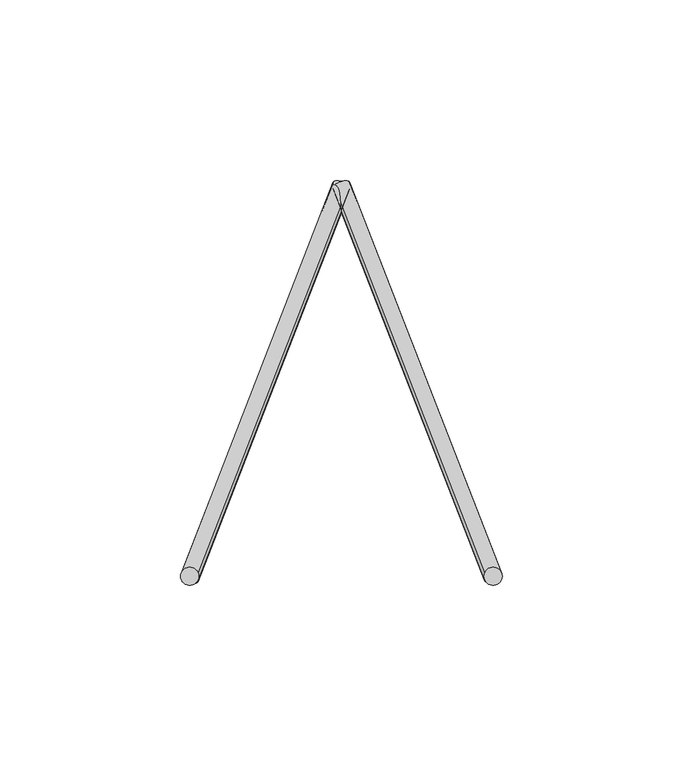
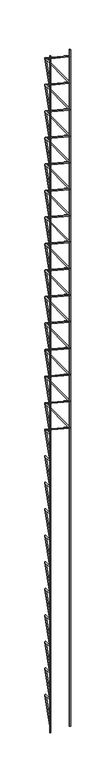
"""IFC4 building model written with IfcOpenShell, lengths in millimetres: proxy geometry, Pre-fab. (Vigota 1 - Pano 3)."""

from ifc_helpers import new_model, si_unit, point, frame, frame_2d, origin, origin_with_axes, origin_2d, place, context, project, spatial, circle_curve, trimmed, segment, composite_curve, outline, extrude, source, transform, mapped, element, save


def structural_framing_81210333(model_context):
    return source(origin(), model_context, "Body", "SweptSolid", [
        extrude(outline(composite_curve([segment(trimmed(circle_curve(origin_2d(), 2.5), [point((2.5, 0.0))], [point((-2.5, 0.0))], False, "CARTESIAN"), True, "CONTINUOUS"), segment(trimmed(circle_curve(origin_2d(), 2.5), [point((-2.5, 0.0))], [point((2.5, 0.0))], False, "CARTESIAN"), True, "CONTINUOUS")], self_intersect=False)), frame((-42.0, 108.0, 1289.500535), z_axis=(0.3218603428886276, -0.8276408817707567, 0.4598004898837537), x_axis=(0.8192319205108605, -3.936835275445103e-11, -0.5734623443750141)), (0.0, 0.0, 1.0), 130.491379),
        extrude(outline(composite_curve([segment(trimmed(circle_curve(origin_2d(), 2.5), [point((2.5, 0.0))], [point((-2.5, 0.0))], False, "CARTESIAN"), True, "CONTINUOUS"), segment(trimmed(circle_curve(origin_2d(), 2.5), [point((-2.5, 0.0))], [point((2.5, 0.0))], False, "CARTESIAN"), True, "CONTINUOUS")], self_intersect=False)), frame((0.0, 0.0, 1349.500535), z_axis=(-0.3218603428886276, 0.8276408817707567, 0.4598004898837537), x_axis=(0.8192319205108605, -3.936835275445103e-11, 0.5734623443750141)), (0.0, 0.0, 1.0), 130.491379),
        extrude(outline(composite_curve([segment(trimmed(circle_curve(origin_2d(), 2.5), [point((2.5, 0.0))], [point((-2.5, 0.0))], False, "CARTESIAN"), True, "CONTINUOUS"), segment(trimmed(circle_curve(origin_2d(), 2.5), [point((-2.5, 0.0))], [point((2.5, 0.0))], False, "CARTESIAN"), True, "CONTINUOUS")], self_intersect=False)), frame((-42.0, 108.0, 1409.500535), z_axis=(0.3218603428886276, -0.8276408817707567, 0.4598004898837537), x_axis=(0.8192319205108605, -3.936835275445103e-11, -0.5734623443750141)), (0.0, 0.0, 1.0), 130.491379),
        extrude(outline(composite_curve([segment(trimmed(circle_curve(origin_2d(), 2.5), [point((2.5, 0.0))], [point((-2.5, 0.0))], False, "CARTESIAN"), True, "CONTINUOUS"), segment(trimmed(circle_curve(origin_2d(), 2.5), [point((-2.5, 0.0))], [point((2.5, 0.0))], False, "CARTESIAN"), True, "CONTINUOUS")], self_intersect=False)), frame((0.0, 0.0, 1469.500535), z_axis=(-0.3218603428886276, 0.8276408817707567, 0.4598004898837537), x_axis=(0.8192319205108605, -3.936835275445103e-11, 0.5734623443750141)), (0.0, 0.0, 1.0), 130.491379),
        extrude(outline(composite_curve([segment(trimmed(circle_curve(origin_2d(), 2.5), [point((2.5, 0.0))], [point((-2.5, 0.0))], False, "CARTESIAN"), True, "CONTINUOUS"), segment(trimmed(circle_curve(origin_2d(), 2.5), [point((-2.5, 0.0))], [point((2.5, 0.0))], False, "CARTESIAN"), True, "CONTINUOUS")], self_intersect=False)), frame((-42.0, 108.0, 1529.500535), z_axis=(0.3218603428886276, -0.8276408817707567, 0.4598004898837537), x_axis=(0.8192319205108605, -3.936835275445103e-11, -0.5734623443750141)), (0.0, 0.0, 1.0), 130.491379),
        extrude(outline(composite_curve([segment(trimmed(circle_curve(origin_2d(), 2.5), [point((2.5, 0.0))], [point((-2.5, 0.0))], False, "CARTESIAN"), True, "CONTINUOUS"), segment(trimmed(circle_curve(origin_2d(), 2.5), [point((-2.5, 0.0))], [point((2.5, 0.0))], False, "CARTESIAN"), True, "CONTINUOUS")], self_intersect=False)), frame((0.0, 0.0, 1589.500535), z_axis=(-0.3218603428886276, 0.8276408817707567, 0.4598004898837537), x_axis=(0.8192319205108605, -3.936835275445103e-11, 0.5734623443750141)), (0.0, 0.0, 1.0), 130.491379),
        extrude(outline(composite_curve([segment(trimmed(circle_curve(origin_2d(), 2.5), [point((2.5, 0.0))], [point((-2.5, 0.0))], False, "CARTESIAN"), True, "CONTINUOUS"), segment(trimmed(circle_curve(origin_2d(), 2.5), [point((-2.5, 0.0))], [point((2.5, 0.0))], False, "CARTESIAN"), True, "CONTINUOUS")], self_intersect=False)), frame((-42.0, 108.0, 1649.500535), z_axis=(0.3218603428886276, -0.8276408817707567, 0.4598004898837537), x_axis=(0.8192319205108605, -3.936835275445103e-11, -0.5734623443750141)), (0.0, 0.0, 1.0), 130.491379),
        extrude(outline(composite_curve([segment(trimmed(circle_curve(origin_2d(), 2.5), [point((2.5, 0.0))], [point((-2.5, 0.0))], False, "CARTESIAN"), True, "CONTINUOUS"), segment(trimmed(circle_curve(origin_2d(), 2.5), [point((-2.5, 0.0))], [point((2.5, 0.0))], False, "CARTESIAN"), True, "CONTINUOUS")], self_intersect=False)), frame((0.0, 0.0, 1709.500535), z_axis=(-0.3218603428886276, 0.8276408817707567, 0.4598004898837537), x_axis=(0.8192319205108605, -3.936835275445103e-11, 0.5734623443750141)), (0.0, 0.0, 1.0), 130.491379),
        extrude(outline(composite_curve([segment(trimmed(circle_curve(origin_2d(), 2.5), [point((2.5, 0.0))], [point((-2.5, 0.0))], False, "CARTESIAN"), True, "CONTINUOUS"), segment(trimmed(circle_curve(origin_2d(), 2.5), [point((-2.5, 0.0))], [point((2.5, 0.0))], False, "CARTESIAN"), True, "CONTINUOUS")], self_intersect=False)), frame((-42.0, 108.0, 1769.500535), z_axis=(0.3218603428886276, -0.8276408817707567, 0.4598004898837537), x_axis=(0.8192319205108605, -3.936835275445103e-11, -0.5734623443750141)), (0.0, 0.0, 1.0), 130.491379),
        extrude(outline(composite_curve([segment(trimmed(circle_curve(origin_2d(), 2.5), [point((2.5, 0.0))], [point((-2.5, 0.0))], False, "CARTESIAN"), True, "CONTINUOUS"), segment(trimmed(circle_curve(origin_2d(), 2.5), [point((-2.5, 0.0))], [point((2.5, 0.0))], False, "CARTESIAN"), True, "CONTINUOUS")], self_intersect=False)), frame((0.0, 0.0, 1829.500535), z_axis=(-0.3218603428886276, 0.8276408817707567, 0.4598004898837537), x_axis=(0.8192319205108605, -3.936835275445103e-11, 0.5734623443750141)), (0.0, 0.0, 1.0), 130.491379),
        extrude(outline(composite_curve([segment(trimmed(circle_curve(origin_2d(), 2.5), [point((2.5, 0.0))], [point((-2.5, 0.0))], False, "CARTESIAN"), True, "CONTINUOUS"), segment(trimmed(circle_curve(origin_2d(), 2.5), [point((-2.5, 0.0))], [point((2.5, 0.0))], False, "CARTESIAN"), True, "CONTINUOUS")], self_intersect=False)), frame((-42.0, 108.0, 1889.500535), z_axis=(0.3218603428886276, -0.8276408817707567, 0.4598004898837537), x_axis=(0.8192319205108605, -3.936835275445103e-11, -0.5734623443750141)), (0.0, 0.0, 1.0), 130.491379),
        extrude(outline(composite_curve([segment(trimmed(circle_curve(origin_2d(), 2.5), [point((2.5, 0.0))], [point((-2.5, 0.0))], False, "CARTESIAN"), True, "CONTINUOUS"), segment(trimmed(circle_curve(origin_2d(), 2.5), [point((-2.5, 0.0))], [point((2.5, 0.0))], False, "CARTESIAN"), True, "CONTINUOUS")], self_intersect=False)), frame((0.0, 0.0, 1949.500535), z_axis=(-0.3218603428886276, 0.8276408817707567, 0.4598004898837537), x_axis=(0.8192319205108605, -3.936835275445103e-11, 0.5734623443750141)), (0.0, 0.0, 1.0), 130.491379),
        extrude(outline(composite_curve([segment(trimmed(circle_curve(origin_2d(), 2.5), [point((2.5, 0.0))], [point((-2.5, 0.0))], False, "CARTESIAN"), True, "CONTINUOUS"), segment(trimmed(circle_curve(origin_2d(), 2.5), [point((-2.5, 0.0))], [point((2.5, 0.0))], False, "CARTESIAN"), True, "CONTINUOUS")], self_intersect=False)), frame((-42.0, 108.0, 2009.500535), z_axis=(0.3218603428886276, -0.8276408817707567, 0.4598004898837537), x_axis=(0.8192319205108605, -3.936835275445103e-11, -0.5734623443750141)), (0.0, 0.0, 1.0), 130.491379),
        extrude(outline(composite_curve([segment(trimmed(circle_curve(origin_2d(), 2.5), [point((2.5, 0.0))], [point((-2.5, 0.0))], False, "CARTESIAN"), True, "CONTINUOUS"), segment(trimmed(circle_curve(origin_2d(), 2.5), [point((-2.5, 0.0))], [point((2.5, 0.0))], False, "CARTESIAN"), True, "CONTINUOUS")], self_intersect=False)), frame((0.0, 0.0, 2069.500535), z_axis=(-0.3218603428886276, 0.8276408817707567, 0.4598004898837537), x_axis=(0.8192319205108605, -3.936835275445103e-11, 0.5734623443750141)), (0.0, 0.0, 1.0), 130.491379),
        extrude(outline(composite_curve([segment(trimmed(circle_curve(origin_2d(), 2.5), [point((2.5, 0.0))], [point((-2.5, 0.0))], False, "CARTESIAN"), True, "CONTINUOUS"), segment(trimmed(circle_curve(origin_2d(), 2.5), [point((-2.5, 0.0))], [point((2.5, 0.0))], False, "CARTESIAN"), True, "CONTINUOUS")], self_intersect=False)), frame((-42.0, 108.0, 2129.500535), z_axis=(0.3218603428886276, -0.8276408817707567, 0.4598004898837537), x_axis=(0.8192319205108605, -3.936835275445103e-11, -0.5734623443750141)), (0.0, 0.0, 1.0), 130.491379),
        extrude(outline(composite_curve([segment(trimmed(circle_curve(origin_2d(), 2.5), [point((2.5, 0.0))], [point((-2.5, 0.0))], False, "CARTESIAN"), True, "CONTINUOUS"), segment(trimmed(circle_curve(origin_2d(), 2.5), [point((-2.5, 0.0))], [point((2.5, 0.0))], False, "CARTESIAN"), True, "CONTINUOUS")], self_intersect=False)), frame((0.0, 0.0, 2189.500535), z_axis=(-0.3218603428886276, 0.8276408817707567, 0.4598004898837537), x_axis=(0.8192319205108605, -3.936835275445103e-11, 0.5734623443750141)), (0.0, 0.0, 1.0), 130.491379),
        extrude(outline(composite_curve([segment(trimmed(circle_curve(origin_2d(), 2.5), [point((2.5, 0.0))], [point((-2.5, 0.0))], False, "CARTESIAN"), True, "CONTINUOUS"), segment(trimmed(circle_curve(origin_2d(), 2.5), [point((-2.5, 0.0))], [point((2.5, 0.0))], False, "CARTESIAN"), True, "CONTINUOUS")], self_intersect=False)), frame((-42.0, 108.0, 2249.500535), z_axis=(0.3218603428886276, -0.8276408817707567, 0.4598004898837537), x_axis=(0.8192319205108605, -3.936835275445103e-11, -0.5734623443750141)), (0.0, 0.0, 1.0), 130.491379),
        extrude(outline(composite_curve([segment(trimmed(circle_curve(origin_2d(), 2.5), [point((2.5, 0.0))], [point((-2.5, 0.0))], False, "CARTESIAN"), True, "CONTINUOUS"), segment(trimmed(circle_curve(origin_2d(), 2.5), [point((-2.5, 0.0))], [point((2.5, 0.0))], False, "CARTESIAN"), True, "CONTINUOUS")], self_intersect=False)), frame((0.0, 0.0, 2309.500535), z_axis=(-0.3218603428886276, 0.8276408817707567, 0.4598004898837537), x_axis=(0.8192319205108605, -3.936835275445103e-11, 0.5734623443750141)), (0.0, 0.0, 1.0), 130.491379),
        extrude(outline(composite_curve([segment(trimmed(circle_curve(origin_2d(), 2.5), [point((2.5, 0.0))], [point((-2.5, 0.0))], False, "CARTESIAN"), True, "CONTINUOUS"), segment(trimmed(circle_curve(origin_2d(), 2.5), [point((-2.5, 0.0))], [point((2.5, 0.0))], False, "CARTESIAN"), True, "CONTINUOUS")], self_intersect=False)), frame((-42.0, 108.0, 2369.500535), z_axis=(0.3218603428886276, -0.8276408817707567, 0.4598004898837537), x_axis=(0.8192319205108605, -3.936835275445103e-11, -0.5734623443750141)), (0.0, 0.0, 1.0), 130.491379),
        extrude(outline(composite_curve([segment(trimmed(circle_curve(origin_2d(), 2.5), [point((2.5, 0.0))], [point((-2.5, 0.0))], False, "CARTESIAN"), True, "CONTINUOUS"), segment(trimmed(circle_curve(origin_2d(), 2.5), [point((-2.5, 0.0))], [point((2.5, 0.0))], False, "CARTESIAN"), True, "CONTINUOUS")], self_intersect=False)), frame((0.0, 0.0, 2429.500535), z_axis=(-0.3218603428886276, 0.8276408817707567, 0.4598004898837537), x_axis=(0.8192319205108605, -3.936835275445103e-11, 0.5734623443750141)), (0.0, 0.0, 1.0), 130.491379),
        extrude(outline(composite_curve([segment(trimmed(circle_curve(origin_2d(), 2.5), [point((2.5, 0.0))], [point((-2.5, 0.0))], False, "CARTESIAN"), True, "CONTINUOUS"), segment(trimmed(circle_curve(origin_2d(), 2.5), [point((-2.5, 0.0))], [point((2.5, 0.0))], False, "CARTESIAN"), True, "CONTINUOUS")], self_intersect=False)), frame((-42.0, 108.0, 2489.500535), z_axis=(0.3218603428886276, -0.8276408817707567, 0.4598004898837537), x_axis=(0.8192319205108605, -3.936835275445103e-11, -0.5734623443750141)), (0.0, 0.0, 1.0), 130.491379),
        extrude(outline(composite_curve([segment(trimmed(circle_curve(origin_2d(), 2.5), [point((2.5, 0.0))], [point((-2.5, 0.0))], False, "CARTESIAN"), True, "CONTINUOUS"), segment(trimmed(circle_curve(origin_2d(), 2.5), [point((-2.5, 0.0))], [point((2.5, 0.0))], False, "CARTESIAN"), True, "CONTINUOUS")], self_intersect=False)), frame((0.0, 0.0, 2549.500535), z_axis=(-0.3218603428886276, 0.8276408817707567, 0.4598004898837537), x_axis=(0.8192319205108605, -3.936835275445103e-11, 0.5734623443750141)), (0.0, 0.0, 1.0), 130.491379),
        extrude(outline(composite_curve([segment(trimmed(circle_curve(origin_2d(), 2.5), [point((2.5, 0.0))], [point((-2.5, 0.0))], False, "CARTESIAN"), True, "CONTINUOUS"), segment(trimmed(circle_curve(origin_2d(), 2.5), [point((-2.5, 0.0))], [point((2.5, 0.0))], False, "CARTESIAN"), True, "CONTINUOUS")], self_intersect=False)), frame((-42.0, 108.0, 2609.500535), z_axis=(0.3218603428886276, -0.8276408817707567, 0.4598004898837537), x_axis=(0.8192319205108605, -3.936835275445103e-11, -0.5734623443750141)), (0.0, 0.0, 1.0), 130.491379),
        extrude(outline(composite_curve([segment(trimmed(circle_curve(origin_2d(), 2.5), [point((2.5, 0.0))], [point((-2.5, 0.0))], False, "CARTESIAN"), True, "CONTINUOUS"), segment(trimmed(circle_curve(origin_2d(), 2.5), [point((-2.5, 0.0))], [point((2.5, 0.0))], False, "CARTESIAN"), True, "CONTINUOUS")], self_intersect=False)), frame((0.0, 0.0, 2669.500535), z_axis=(-0.3218603428886276, 0.8276408817707567, 0.4598004898837537), x_axis=(0.8192319205108605, -3.936835275445103e-11, 0.5734623443750141)), (0.0, 0.0, 1.0), 130.491379),
        extrude(outline(composite_curve([segment(trimmed(circle_curve(origin_2d(), 2.5), [point((2.5, 0.0))], [point((-2.5, 0.0))], False, "CARTESIAN"), True, "CONTINUOUS"), segment(trimmed(circle_curve(origin_2d(), 2.5), [point((-2.5, 0.0))], [point((2.5, 0.0))], False, "CARTESIAN"), True, "CONTINUOUS")], self_intersect=False)), frame((-42.0, 108.0, 2729.500535), z_axis=(0.3218603428886276, -0.8276408817707567, 0.4598004898837537), x_axis=(0.8192319205108605, -3.936835275445103e-11, -0.5734623443750141)), (0.0, 0.0, 1.0), 130.491379),
        extrude(outline(composite_curve([segment(trimmed(circle_curve(origin_2d(), 2.5), [point((2.5, 0.0))], [point((-2.5, 0.0))], False, "CARTESIAN"), True, "CONTINUOUS"), segment(trimmed(circle_curve(origin_2d(), 2.5), [point((-2.5, 0.0))], [point((2.5, 0.0))], False, "CARTESIAN"), True, "CONTINUOUS")], self_intersect=False)), frame((0.0, 0.0, 2789.500535), z_axis=(-0.3218603428886276, 0.8276408817707567, 0.4598004898837537), x_axis=(0.8192319205108605, -3.936835275445103e-11, 0.5734623443750141)), (0.0, 0.0, 1.0), 130.491379),
        extrude(outline(composite_curve([segment(trimmed(circle_curve(origin_2d(), 2.5), [point((2.5, 0.0))], [point((-2.5, 0.0))], False, "CARTESIAN"), True, "CONTINUOUS"), segment(trimmed(circle_curve(origin_2d(), 2.5), [point((-2.5, 0.0))], [point((2.5, 0.0))], False, "CARTESIAN"), True, "CONTINUOUS")], self_intersect=False)), frame((-42.0, 108.0, 2849.500535), z_axis=(0.3218603428886276, -0.8276408817707567, 0.4598004898837537), x_axis=(0.8192319205108605, -3.936835275445103e-11, -0.5734623443750141)), (0.0, 0.0, 1.0), 130.491379),
        extrude(outline(composite_curve([segment(trimmed(circle_curve(origin_2d(), 2.5), [point((2.5, 0.0))], [point((-2.5, 0.0))], False, "CARTESIAN"), True, "CONTINUOUS"), segment(trimmed(circle_curve(origin_2d(), 2.5), [point((-2.5, 0.0))], [point((2.5, 0.0))], False, "CARTESIAN"), True, "CONTINUOUS")], self_intersect=False)), frame((0.0, 0.0, 2909.500535), z_axis=(-0.3218603428886276, 0.8276408817707567, 0.4598004898837537), x_axis=(0.8192319205108605, -3.936835275445103e-11, 0.5734623443750141)), (0.0, 0.0, 1.0), 130.491379),
        extrude(outline(composite_curve([segment(trimmed(circle_curve(origin_2d(), 2.5), [point((2.5, 0.0))], [point((-2.5, 0.0))], False, "CARTESIAN"), True, "CONTINUOUS"), segment(trimmed(circle_curve(origin_2d(), 2.5), [point((-2.5, 0.0))], [point((2.5, 0.0))], False, "CARTESIAN"), True, "CONTINUOUS")], self_intersect=False)), frame((-42.0, 108.0, 2969.500535), z_axis=(0.3218603428886276, -0.8276408817707567, 0.4598004898837537), x_axis=(0.8192319205108605, -3.936835275445103e-11, -0.5734623443750141)), (0.0, 0.0, 1.0), 130.491379),
        extrude(outline(composite_curve([segment(trimmed(circle_curve(frame_2d((-84.0, 0.0)), 2.5), [point((-81.5, 0.0))], [point((-86.5, 0.0))], False, "CARTESIAN"), True, "CONTINUOUS"), segment(trimmed(circle_curve(frame_2d((-84.0, 0.0)), 2.5), [point((-86.5, 0.0))], [point((-81.5, 0.0))], False, "CARTESIAN"), True, "CONTINUOUS")], self_intersect=False)), origin_with_axes(), (0.0, 0.0, 1.0), 3059.00107),
        extrude(outline(composite_curve([segment(trimmed(circle_curve(origin_2d(), 2.5), [point((2.5, 0.0))], [point((-2.5, 0.0))], False, "CARTESIAN"), True, "CONTINUOUS"), segment(trimmed(circle_curve(origin_2d(), 2.5), [point((-2.5, 0.0))], [point((2.5, 0.0))], False, "CARTESIAN"), True, "CONTINUOUS")], self_intersect=False)), frame((-84.0, 0.0, 29.500535), z_axis=(0.3218603428886276, 0.8276408817707567, 0.4598004898837537), x_axis=(0.8192319205108605, 3.936835275445103e-11, -0.5734623443750141)), (0.0, 0.0, 1.0), 130.491379),
        extrude(outline(composite_curve([segment(trimmed(circle_curve(origin_2d(), 2.5), [point((2.5, 0.0))], [point((-2.5, 0.0))], False, "CARTESIAN"), True, "CONTINUOUS"), segment(trimmed(circle_curve(origin_2d(), 2.5), [point((-2.5, 0.0))], [point((2.5, 0.0))], False, "CARTESIAN"), True, "CONTINUOUS")], self_intersect=False)), frame((-42.0, 108.0, 89.500535), z_axis=(-0.3218603428886276, -0.8276408817707567, 0.4598004898837537), x_axis=(0.8192319205108605, 3.936835275445103e-11, 0.5734623443750141)), (0.0, 0.0, 1.0), 130.491379),
        extrude(outline(composite_curve([segment(trimmed(circle_curve(origin_2d(), 2.5), [point((2.5, 0.0))], [point((-2.5, 0.0))], False, "CARTESIAN"), True, "CONTINUOUS"), segment(trimmed(circle_curve(origin_2d(), 2.5), [point((-2.5, 0.0))], [point((2.5, 0.0))], False, "CARTESIAN"), True, "CONTINUOUS")], self_intersect=False)), frame((-84.0, 0.0, 149.500535), z_axis=(0.3218603428886276, 0.8276408817707567, 0.4598004898837537), x_axis=(0.8192319205108605, 3.936835275445103e-11, -0.5734623443750141)), (0.0, 0.0, 1.0), 130.491379),
        extrude(outline(composite_curve([segment(trimmed(circle_curve(origin_2d(), 2.5), [point((2.5, 0.0))], [point((-2.5, 0.0))], False, "CARTESIAN"), True, "CONTINUOUS"), segment(trimmed(circle_curve(origin_2d(), 2.5), [point((-2.5, 0.0))], [point((2.5, 0.0))], False, "CARTESIAN"), True, "CONTINUOUS")], self_intersect=False)), frame((-42.0, 108.0, 209.500535), z_axis=(-0.3218603428886276, -0.8276408817707567, 0.4598004898837537), x_axis=(0.8192319205108605, 3.936835275445103e-11, 0.5734623443750141)), (0.0, 0.0, 1.0), 130.491379),
        extrude(outline(composite_curve([segment(trimmed(circle_curve(origin_2d(), 2.5), [point((2.5, 0.0))], [point((-2.5, 0.0))], False, "CARTESIAN"), True, "CONTINUOUS"), segment(trimmed(circle_curve(origin_2d(), 2.5), [point((-2.5, 0.0))], [point((2.5, 0.0))], False, "CARTESIAN"), True, "CONTINUOUS")], self_intersect=False)), frame((-84.0, 0.0, 269.500535), z_axis=(0.3218603428886276, 0.8276408817707567, 0.4598004898837537), x_axis=(0.8192319205108605, 3.936835275445103e-11, -0.5734623443750141)), (0.0, 0.0, 1.0), 130.491379),
        extrude(outline(composite_curve([segment(trimmed(circle_curve(origin_2d(), 2.5), [point((2.5, 0.0))], [point((-2.5, 0.0))], False, "CARTESIAN"), True, "CONTINUOUS"), segment(trimmed(circle_curve(origin_2d(), 2.5), [point((-2.5, 0.0))], [point((2.5, 0.0))], False, "CARTESIAN"), True, "CONTINUOUS")], self_intersect=False)), frame((-42.0, 108.0, 329.500535), z_axis=(-0.3218603428886276, -0.8276408817707567, 0.4598004898837537), x_axis=(0.8192319205108605, 3.936835275445103e-11, 0.5734623443750141)), (0.0, 0.0, 1.0), 130.491379),
        extrude(outline(composite_curve([segment(trimmed(circle_curve(origin_2d(), 2.5), [point((2.5, 0.0))], [point((-2.5, 0.0))], False, "CARTESIAN"), True, "CONTINUOUS"), segment(trimmed(circle_curve(origin_2d(), 2.5), [point((-2.5, 0.0))], [point((2.5, 0.0))], False, "CARTESIAN"), True, "CONTINUOUS")], self_intersect=False)), frame((-84.0, 0.0, 389.500535), z_axis=(0.3218603428886276, 0.8276408817707567, 0.4598004898837537), x_axis=(0.8192319205108605, 3.936835275445103e-11, -0.5734623443750141)), (0.0, 0.0, 1.0), 130.491379),
        extrude(outline(composite_curve([segment(trimmed(circle_curve(origin_2d(), 2.5), [point((2.5, 0.0))], [point((-2.5, 0.0))], False, "CARTESIAN"), True, "CONTINUOUS"), segment(trimmed(circle_curve(origin_2d(), 2.5), [point((-2.5, 0.0))], [point((2.5, 0.0))], False, "CARTESIAN"), True, "CONTINUOUS")], self_intersect=False)), frame((-42.0, 108.0, 449.500535), z_axis=(-0.3218603428886276, -0.8276408817707567, 0.4598004898837537), x_axis=(0.8192319205108605, 3.936835275445103e-11, 0.5734623443750141)), (0.0, 0.0, 1.0), 130.491379),
        extrude(outline(composite_curve([segment(trimmed(circle_curve(origin_2d(), 2.5), [point((2.5, 0.0))], [point((-2.5, 0.0))], False, "CARTESIAN"), True, "CONTINUOUS"), segment(trimmed(circle_curve(origin_2d(), 2.5), [point((-2.5, 0.0))], [point((2.5, 0.0))], False, "CARTESIAN"), True, "CONTINUOUS")], self_intersect=False)), frame((-84.0, 0.0, 509.500535), z_axis=(0.3218603428886276, 0.8276408817707567, 0.4598004898837537), x_axis=(0.8192319205108605, 3.936835275445103e-11, -0.5734623443750141)), (0.0, 0.0, 1.0), 130.491379),
        extrude(outline(composite_curve([segment(trimmed(circle_curve(origin_2d(), 2.5), [point((2.5, 0.0))], [point((-2.5, 0.0))], False, "CARTESIAN"), True, "CONTINUOUS"), segment(trimmed(circle_curve(origin_2d(), 2.5), [point((-2.5, 0.0))], [point((2.5, 0.0))], False, "CARTESIAN"), True, "CONTINUOUS")], self_intersect=False)), frame((-42.0, 108.0, 569.500535), z_axis=(-0.3218603428886276, -0.8276408817707567, 0.4598004898837537), x_axis=(0.8192319205108605, 3.936835275445103e-11, 0.5734623443750141)), (0.0, 0.0, 1.0), 130.491379),
        extrude(outline(composite_curve([segment(trimmed(circle_curve(origin_2d(), 2.5), [point((2.5, 0.0))], [point((-2.5, 0.0))], False, "CARTESIAN"), True, "CONTINUOUS"), segment(trimmed(circle_curve(origin_2d(), 2.5), [point((-2.5, 0.0))], [point((2.5, 0.0))], False, "CARTESIAN"), True, "CONTINUOUS")], self_intersect=False)), frame((-84.0, 0.0, 629.500535), z_axis=(0.3218603428886276, 0.8276408817707567, 0.4598004898837537), x_axis=(0.8192319205108605, 3.936835275445103e-11, -0.5734623443750141)), (0.0, 0.0, 1.0), 130.491379),
        extrude(outline(composite_curve([segment(trimmed(circle_curve(origin_2d(), 2.5), [point((2.5, 0.0))], [point((-2.5, 0.0))], False, "CARTESIAN"), True, "CONTINUOUS"), segment(trimmed(circle_curve(origin_2d(), 2.5), [point((-2.5, 0.0))], [point((2.5, 0.0))], False, "CARTESIAN"), True, "CONTINUOUS")], self_intersect=False)), frame((-42.0, 108.0, 689.500535), z_axis=(-0.3218603428886276, -0.8276408817707567, 0.4598004898837537), x_axis=(0.8192319205108605, 3.936835275445103e-11, 0.5734623443750141)), (0.0, 0.0, 1.0), 130.491379),
        extrude(outline(composite_curve([segment(trimmed(circle_curve(origin_2d(), 2.5), [point((2.5, 0.0))], [point((-2.5, 0.0))], False, "CARTESIAN"), True, "CONTINUOUS"), segment(trimmed(circle_curve(origin_2d(), 2.5), [point((-2.5, 0.0))], [point((2.5, 0.0))], False, "CARTESIAN"), True, "CONTINUOUS")], self_intersect=False)), frame((-84.0, 0.0, 749.500535), z_axis=(0.3218603428886276, 0.8276408817707567, 0.4598004898837537), x_axis=(0.8192319205108605, 3.936835275445103e-11, -0.5734623443750141)), (0.0, 0.0, 1.0), 130.491379),
        extrude(outline(composite_curve([segment(trimmed(circle_curve(origin_2d(), 2.5), [point((2.5, 0.0))], [point((-2.5, 0.0))], False, "CARTESIAN"), True, "CONTINUOUS"), segment(trimmed(circle_curve(origin_2d(), 2.5), [point((-2.5, 0.0))], [point((2.5, 0.0))], False, "CARTESIAN"), True, "CONTINUOUS")], self_intersect=False)), frame((-42.0, 108.0, 809.500535), z_axis=(-0.3218603428886276, -0.8276408817707567, 0.4598004898837537), x_axis=(0.8192319205108605, 3.936835275445103e-11, 0.5734623443750141)), (0.0, 0.0, 1.0), 130.491379),
        extrude(outline(composite_curve([segment(trimmed(circle_curve(origin_2d(), 2.5), [point((2.5, 0.0))], [point((-2.5, 0.0))], False, "CARTESIAN"), True, "CONTINUOUS"), segment(trimmed(circle_curve(origin_2d(), 2.5), [point((-2.5, 0.0))], [point((2.5, 0.0))], False, "CARTESIAN"), True, "CONTINUOUS")], self_intersect=False)), frame((-84.0, 0.0, 869.500535), z_axis=(0.3218603428886276, 0.8276408817707567, 0.4598004898837537), x_axis=(0.8192319205108605, 3.936835275445103e-11, -0.5734623443750141)), (0.0, 0.0, 1.0), 130.491379),
        extrude(outline(composite_curve([segment(trimmed(circle_curve(origin_2d(), 2.5), [point((2.5, 0.0))], [point((-2.5, 0.0))], False, "CARTESIAN"), True, "CONTINUOUS"), segment(trimmed(circle_curve(origin_2d(), 2.5), [point((-2.5, 0.0))], [point((2.5, 0.0))], False, "CARTESIAN"), True, "CONTINUOUS")], self_intersect=False)), frame((-42.0, 108.0, 929.500535), z_axis=(-0.3218603428886276, -0.8276408817707567, 0.4598004898837537), x_axis=(0.8192319205108605, 3.936835275445103e-11, 0.5734623443750141)), (0.0, 0.0, 1.0), 130.491379),
        extrude(outline(composite_curve([segment(trimmed(circle_curve(origin_2d(), 2.5), [point((2.5, 0.0))], [point((-2.5, 0.0))], False, "CARTESIAN"), True, "CONTINUOUS"), segment(trimmed(circle_curve(origin_2d(), 2.5), [point((-2.5, 0.0))], [point((2.5, 0.0))], False, "CARTESIAN"), True, "CONTINUOUS")], self_intersect=False)), frame((-84.0, 0.0, 989.500535), z_axis=(0.3218603428886276, 0.8276408817707567, 0.4598004898837537), x_axis=(0.8192319205108605, 3.936835275445103e-11, -0.5734623443750141)), (0.0, 0.0, 1.0), 130.491379),
        extrude(outline(composite_curve([segment(trimmed(circle_curve(origin_2d(), 2.5), [point((2.5, 0.0))], [point((-2.5, 0.0))], False, "CARTESIAN"), True, "CONTINUOUS"), segment(trimmed(circle_curve(origin_2d(), 2.5), [point((-2.5, 0.0))], [point((2.5, 0.0))], False, "CARTESIAN"), True, "CONTINUOUS")], self_intersect=False)), frame((-42.0, 108.0, 1049.500535), z_axis=(-0.3218603428886276, -0.8276408817707567, 0.4598004898837537), x_axis=(0.8192319205108605, 3.936835275445103e-11, 0.5734623443750141)), (0.0, 0.0, 1.0), 130.491379),
        extrude(outline(composite_curve([segment(trimmed(circle_curve(origin_2d(), 2.5), [point((2.5, 0.0))], [point((-2.5, 0.0))], False, "CARTESIAN"), True, "CONTINUOUS"), segment(trimmed(circle_curve(origin_2d(), 2.5), [point((-2.5, 0.0))], [point((2.5, 0.0))], False, "CARTESIAN"), True, "CONTINUOUS")], self_intersect=False)), frame((-84.0, 0.0, 1109.500535), z_axis=(0.3218603428886276, 0.8276408817707567, 0.4598004898837537), x_axis=(0.8192319205108605, 3.936835275445103e-11, -0.5734623443750141)), (0.0, 0.0, 1.0), 130.491379),
        extrude(outline(composite_curve([segment(trimmed(circle_curve(origin_2d(), 2.5), [point((2.5, 0.0))], [point((-2.5, 0.0))], False, "CARTESIAN"), True, "CONTINUOUS"), segment(trimmed(circle_curve(origin_2d(), 2.5), [point((-2.5, 0.0))], [point((2.5, 0.0))], False, "CARTESIAN"), True, "CONTINUOUS")], self_intersect=False)), frame((-42.0, 108.0, 1169.500535), z_axis=(-0.3218603428886276, -0.8276408817707567, 0.4598004898837537), x_axis=(0.8192319205108605, 3.936835275445103e-11, 0.5734623443750141)), (0.0, 0.0, 1.0), 130.491379),
        extrude(outline(composite_curve([segment(trimmed(circle_curve(origin_2d(), 2.5), [point((2.5, 0.0))], [point((-2.5, 0.0))], False, "CARTESIAN"), True, "CONTINUOUS"), segment(trimmed(circle_curve(origin_2d(), 2.5), [point((-2.5, 0.0))], [point((2.5, 0.0))], False, "CARTESIAN"), True, "CONTINUOUS")], self_intersect=False)), frame((-84.0, 0.0, 1229.500535), z_axis=(0.3218603428886276, 0.8276408817707567, 0.4598004898837537), x_axis=(0.8192319205108605, 3.936835275445103e-11, -0.5734623443750141)), (0.0, 0.0, 1.0), 130.491379),
        extrude(outline(composite_curve([segment(trimmed(circle_curve(origin_2d(), 2.5), [point((2.5, 0.0))], [point((-2.5, 0.0))], False, "CARTESIAN"), True, "CONTINUOUS"), segment(trimmed(circle_curve(origin_2d(), 2.5), [point((-2.5, 0.0))], [point((2.5, 0.0))], False, "CARTESIAN"), True, "CONTINUOUS")], self_intersect=False)), frame((-42.0, 108.0, 1289.500535), z_axis=(-0.3218603428886276, -0.8276408817707567, 0.4598004898837537), x_axis=(0.8192319205108605, 3.936835275445103e-11, 0.5734623443750141)), (0.0, 0.0, 1.0), 130.491379),
        extrude(outline(composite_curve([segment(trimmed(circle_curve(origin_2d(), 2.5), [point((2.5, 0.0))], [point((-2.5, 0.0))], False, "CARTESIAN"), True, "CONTINUOUS"), segment(trimmed(circle_curve(origin_2d(), 2.5), [point((-2.5, 0.0))], [point((2.5, 0.0))], False, "CARTESIAN"), True, "CONTINUOUS")], self_intersect=False)), frame((-84.0, 0.0, 1349.500535), z_axis=(0.3218603428886276, 0.8276408817707567, 0.4598004898837537), x_axis=(0.8192319205108605, 3.936835275445103e-11, -0.5734623443750141)), (0.0, 0.0, 1.0), 130.491379),
        extrude(outline(composite_curve([segment(trimmed(circle_curve(origin_2d(), 2.5), [point((2.5, 0.0))], [point((-2.5, 0.0))], False, "CARTESIAN"), True, "CONTINUOUS"), segment(trimmed(circle_curve(origin_2d(), 2.5), [point((-2.5, 0.0))], [point((2.5, 0.0))], False, "CARTESIAN"), True, "CONTINUOUS")], self_intersect=False)), frame((-42.0, 108.0, 1409.500535), z_axis=(-0.3218603428886276, -0.8276408817707567, 0.4598004898837537), x_axis=(0.8192319205108605, 3.936835275445103e-11, 0.5734623443750141)), (0.0, 0.0, 1.0), 130.491379),
        extrude(outline(composite_curve([segment(trimmed(circle_curve(origin_2d(), 2.5), [point((2.5, 0.0))], [point((-2.5, 0.0))], False, "CARTESIAN"), True, "CONTINUOUS"), segment(trimmed(circle_curve(origin_2d(), 2.5), [point((-2.5, 0.0))], [point((2.5, 0.0))], False, "CARTESIAN"), True, "CONTINUOUS")], self_intersect=False)), frame((-84.0, 0.0, 1469.500535), z_axis=(0.3218603428886276, 0.8276408817707567, 0.4598004898837537), x_axis=(0.8192319205108605, 3.936835275445103e-11, -0.5734623443750141)), (0.0, 0.0, 1.0), 130.491379),
        extrude(outline(composite_curve([segment(trimmed(circle_curve(origin_2d(), 2.5), [point((2.5, 0.0))], [point((-2.5, 0.0))], False, "CARTESIAN"), True, "CONTINUOUS"), segment(trimmed(circle_curve(origin_2d(), 2.5), [point((-2.5, 0.0))], [point((2.5, 0.0))], False, "CARTESIAN"), True, "CONTINUOUS")], self_intersect=False)), frame((-42.0, 108.0, 1529.500535), z_axis=(-0.3218603428886276, -0.8276408817707567, 0.4598004898837537), x_axis=(0.8192319205108605, 3.936835275445103e-11, 0.5734623443750141)), (0.0, 0.0, 1.0), 130.491379),
        extrude(outline(composite_curve([segment(trimmed(circle_curve(origin_2d(), 2.5), [point((2.5, 0.0))], [point((-2.5, 0.0))], False, "CARTESIAN"), True, "CONTINUOUS"), segment(trimmed(circle_curve(origin_2d(), 2.5), [point((-2.5, 0.0))], [point((2.5, 0.0))], False, "CARTESIAN"), True, "CONTINUOUS")], self_intersect=False)), frame((-84.0, 0.0, 1589.500535), z_axis=(0.3218603428886276, 0.8276408817707567, 0.4598004898837537), x_axis=(0.8192319205108605, 3.936835275445103e-11, -0.5734623443750141)), (0.0, 0.0, 1.0), 130.491379),
        extrude(outline(composite_curve([segment(trimmed(circle_curve(origin_2d(), 2.5), [point((2.5, 0.0))], [point((-2.5, 0.0))], False, "CARTESIAN"), True, "CONTINUOUS"), segment(trimmed(circle_curve(origin_2d(), 2.5), [point((-2.5, 0.0))], [point((2.5, 0.0))], False, "CARTESIAN"), True, "CONTINUOUS")], self_intersect=False)), frame((-42.0, 108.0, 1649.500535), z_axis=(-0.3218603428886276, -0.8276408817707567, 0.4598004898837537), x_axis=(0.8192319205108605, 3.936835275445103e-11, 0.5734623443750141)), (0.0, 0.0, 1.0), 130.491379),
        extrude(outline(composite_curve([segment(trimmed(circle_curve(origin_2d(), 2.5), [point((2.5, 0.0))], [point((-2.5, 0.0))], False, "CARTESIAN"), True, "CONTINUOUS"), segment(trimmed(circle_curve(origin_2d(), 2.5), [point((-2.5, 0.0))], [point((2.5, 0.0))], False, "CARTESIAN"), True, "CONTINUOUS")], self_intersect=False)), frame((-84.0, 0.0, 1709.500535), z_axis=(0.3218603428886276, 0.8276408817707567, 0.4598004898837537), x_axis=(0.8192319205108605, 3.936835275445103e-11, -0.5734623443750141)), (0.0, 0.0, 1.0), 130.491379),
        extrude(outline(composite_curve([segment(trimmed(circle_curve(origin_2d(), 2.5), [point((2.5, 0.0))], [point((-2.5, 0.0))], False, "CARTESIAN"), True, "CONTINUOUS"), segment(trimmed(circle_curve(origin_2d(), 2.5), [point((-2.5, 0.0))], [point((2.5, 0.0))], False, "CARTESIAN"), True, "CONTINUOUS")], self_intersect=False)), frame((-42.0, 108.0, 1769.500535), z_axis=(-0.3218603428886276, -0.8276408817707567, 0.4598004898837537), x_axis=(0.8192319205108605, 3.936835275445103e-11, 0.5734623443750141)), (0.0, 0.0, 1.0), 130.491379),
        extrude(outline(composite_curve([segment(trimmed(circle_curve(origin_2d(), 2.5), [point((2.5, 0.0))], [point((-2.5, 0.0))], False, "CARTESIAN"), True, "CONTINUOUS"), segment(trimmed(circle_curve(origin_2d(), 2.5), [point((-2.5, 0.0))], [point((2.5, 0.0))], False, "CARTESIAN"), True, "CONTINUOUS")], self_intersect=False)), frame((-84.0, 0.0, 1829.500535), z_axis=(0.3218603428886276, 0.8276408817707567, 0.4598004898837537), x_axis=(0.8192319205108605, 3.936835275445103e-11, -0.5734623443750141)), (0.0, 0.0, 1.0), 130.491379),
        extrude(outline(composite_curve([segment(trimmed(circle_curve(origin_2d(), 2.5), [point((2.5, 0.0))], [point((-2.5, 0.0))], False, "CARTESIAN"), True, "CONTINUOUS"), segment(trimmed(circle_curve(origin_2d(), 2.5), [point((-2.5, 0.0))], [point((2.5, 0.0))], False, "CARTESIAN"), True, "CONTINUOUS")], self_intersect=False)), frame((-42.0, 108.0, 1889.500535), z_axis=(-0.3218603428886276, -0.8276408817707567, 0.4598004898837537), x_axis=(0.8192319205108605, 3.936835275445103e-11, 0.5734623443750141)), (0.0, 0.0, 1.0), 130.491379),
        extrude(outline(composite_curve([segment(trimmed(circle_curve(origin_2d(), 2.5), [point((2.5, 0.0))], [point((-2.5, 0.0))], False, "CARTESIAN"), True, "CONTINUOUS"), segment(trimmed(circle_curve(origin_2d(), 2.5), [point((-2.5, 0.0))], [point((2.5, 0.0))], False, "CARTESIAN"), True, "CONTINUOUS")], self_intersect=False)), frame((-84.0, 0.0, 1949.500535), z_axis=(0.3218603428886276, 0.8276408817707567, 0.4598004898837537), x_axis=(0.8192319205108605, 3.936835275445103e-11, -0.5734623443750141)), (0.0, 0.0, 1.0), 130.491379),
        extrude(outline(composite_curve([segment(trimmed(circle_curve(origin_2d(), 2.5), [point((2.5, 0.0))], [point((-2.5, 0.0))], False, "CARTESIAN"), True, "CONTINUOUS"), segment(trimmed(circle_curve(origin_2d(), 2.5), [point((-2.5, 0.0))], [point((2.5, 0.0))], False, "CARTESIAN"), True, "CONTINUOUS")], self_intersect=False)), frame((-42.0, 108.0, 2009.500535), z_axis=(-0.3218603428886276, -0.8276408817707567, 0.4598004898837537), x_axis=(0.8192319205108605, 3.936835275445103e-11, 0.5734623443750141)), (0.0, 0.0, 1.0), 130.491379),
        extrude(outline(composite_curve([segment(trimmed(circle_curve(origin_2d(), 2.5), [point((2.5, 0.0))], [point((-2.5, 0.0))], False, "CARTESIAN"), True, "CONTINUOUS"), segment(trimmed(circle_curve(origin_2d(), 2.5), [point((-2.5, 0.0))], [point((2.5, 0.0))], False, "CARTESIAN"), True, "CONTINUOUS")], self_intersect=False)), frame((-84.0, 0.0, 2069.500535), z_axis=(0.3218603428886276, 0.8276408817707567, 0.4598004898837537), x_axis=(0.8192319205108605, 3.936835275445103e-11, -0.5734623443750141)), (0.0, 0.0, 1.0), 130.491379),
        extrude(outline(composite_curve([segment(trimmed(circle_curve(origin_2d(), 2.5), [point((2.5, 0.0))], [point((-2.5, 0.0))], False, "CARTESIAN"), True, "CONTINUOUS"), segment(trimmed(circle_curve(origin_2d(), 2.5), [point((-2.5, 0.0))], [point((2.5, 0.0))], False, "CARTESIAN"), True, "CONTINUOUS")], self_intersect=False)), frame((-42.0, 108.0, 2129.500535), z_axis=(-0.3218603428886276, -0.8276408817707567, 0.4598004898837537), x_axis=(0.8192319205108605, 3.936835275445103e-11, 0.5734623443750141)), (0.0, 0.0, 1.0), 130.491379),
        extrude(outline(composite_curve([segment(trimmed(circle_curve(origin_2d(), 2.5), [point((2.5, 0.0))], [point((-2.5, 0.0))], False, "CARTESIAN"), True, "CONTINUOUS"), segment(trimmed(circle_curve(origin_2d(), 2.5), [point((-2.5, 0.0))], [point((2.5, 0.0))], False, "CARTESIAN"), True, "CONTINUOUS")], self_intersect=False)), frame((-84.0, 0.0, 2189.500535), z_axis=(0.3218603428886276, 0.8276408817707567, 0.4598004898837537), x_axis=(0.8192319205108605, 3.936835275445103e-11, -0.5734623443750141)), (0.0, 0.0, 1.0), 130.491379),
        extrude(outline(composite_curve([segment(trimmed(circle_curve(origin_2d(), 2.5), [point((2.5, 0.0))], [point((-2.5, 0.0))], False, "CARTESIAN"), True, "CONTINUOUS"), segment(trimmed(circle_curve(origin_2d(), 2.5), [point((-2.5, 0.0))], [point((2.5, 0.0))], False, "CARTESIAN"), True, "CONTINUOUS")], self_intersect=False)), frame((-42.0, 108.0, 2249.500535), z_axis=(-0.3218603428886276, -0.8276408817707567, 0.4598004898837537), x_axis=(0.8192319205108605, 3.936835275445103e-11, 0.5734623443750141)), (0.0, 0.0, 1.0), 130.491379),
        extrude(outline(composite_curve([segment(trimmed(circle_curve(origin_2d(), 2.5), [point((2.5, 0.0))], [point((-2.5, 0.0))], False, "CARTESIAN"), True, "CONTINUOUS"), segment(trimmed(circle_curve(origin_2d(), 2.5), [point((-2.5, 0.0))], [point((2.5, 0.0))], False, "CARTESIAN"), True, "CONTINUOUS")], self_intersect=False)), frame((-84.0, 0.0, 2309.500535), z_axis=(0.3218603428886276, 0.8276408817707567, 0.4598004898837537), x_axis=(0.8192319205108605, 3.936835275445103e-11, -0.5734623443750141)), (0.0, 0.0, 1.0), 130.491379),
        extrude(outline(composite_curve([segment(trimmed(circle_curve(origin_2d(), 2.5), [point((2.5, 0.0))], [point((-2.5, 0.0))], False, "CARTESIAN"), True, "CONTINUOUS"), segment(trimmed(circle_curve(origin_2d(), 2.5), [point((-2.5, 0.0))], [point((2.5, 0.0))], False, "CARTESIAN"), True, "CONTINUOUS")], self_intersect=False)), frame((-42.0, 108.0, 2369.500535), z_axis=(-0.3218603428886276, -0.8276408817707567, 0.4598004898837537), x_axis=(0.8192319205108605, 3.936835275445103e-11, 0.5734623443750141)), (0.0, 0.0, 1.0), 130.491379),
        extrude(outline(composite_curve([segment(trimmed(circle_curve(origin_2d(), 2.5), [point((2.5, 0.0))], [point((-2.5, 0.0))], False, "CARTESIAN"), True, "CONTINUOUS"), segment(trimmed(circle_curve(origin_2d(), 2.5), [point((-2.5, 0.0))], [point((2.5, 0.0))], False, "CARTESIAN"), True, "CONTINUOUS")], self_intersect=False)), frame((-84.0, 0.0, 2429.500535), z_axis=(0.3218603428886276, 0.8276408817707567, 0.4598004898837537), x_axis=(0.8192319205108605, 3.936835275445103e-11, -0.5734623443750141)), (0.0, 0.0, 1.0), 130.491379),
        extrude(outline(composite_curve([segment(trimmed(circle_curve(origin_2d(), 2.5), [point((2.5, 0.0))], [point((-2.5, 0.0))], False, "CARTESIAN"), True, "CONTINUOUS"), segment(trimmed(circle_curve(origin_2d(), 2.5), [point((-2.5, 0.0))], [point((2.5, 0.0))], False, "CARTESIAN"), True, "CONTINUOUS")], self_intersect=False)), frame((-42.0, 108.0, 2489.500535), z_axis=(-0.3218603428886276, -0.8276408817707567, 0.4598004898837537), x_axis=(0.8192319205108605, 3.936835275445103e-11, 0.5734623443750141)), (0.0, 0.0, 1.0), 130.491379),
        extrude(outline(composite_curve([segment(trimmed(circle_curve(origin_2d(), 2.5), [point((2.5, 0.0))], [point((-2.5, 0.0))], False, "CARTESIAN"), True, "CONTINUOUS"), segment(trimmed(circle_curve(origin_2d(), 2.5), [point((-2.5, 0.0))], [point((2.5, 0.0))], False, "CARTESIAN"), True, "CONTINUOUS")], self_intersect=False)), frame((-84.0, 0.0, 2549.500535), z_axis=(0.3218603428886276, 0.8276408817707567, 0.4598004898837537), x_axis=(0.8192319205108605, 3.936835275445103e-11, -0.5734623443750141)), (0.0, 0.0, 1.0), 130.491379),
        extrude(outline(composite_curve([segment(trimmed(circle_curve(origin_2d(), 2.5), [point((2.5, 0.0))], [point((-2.5, 0.0))], False, "CARTESIAN"), True, "CONTINUOUS"), segment(trimmed(circle_curve(origin_2d(), 2.5), [point((-2.5, 0.0))], [point((2.5, 0.0))], False, "CARTESIAN"), True, "CONTINUOUS")], self_intersect=False)), frame((-42.0, 108.0, 2609.500535), z_axis=(-0.3218603428886276, -0.8276408817707567, 0.4598004898837537), x_axis=(0.8192319205108605, 3.936835275445103e-11, 0.5734623443750141)), (0.0, 0.0, 1.0), 130.491379),
        extrude(outline(composite_curve([segment(trimmed(circle_curve(origin_2d(), 2.5), [point((2.5, 0.0))], [point((-2.5, 0.0))], False, "CARTESIAN"), True, "CONTINUOUS"), segment(trimmed(circle_curve(origin_2d(), 2.5), [point((-2.5, 0.0))], [point((2.5, 0.0))], False, "CARTESIAN"), True, "CONTINUOUS")], self_intersect=False)), frame((-84.0, 0.0, 2669.500535), z_axis=(0.3218603428886276, 0.8276408817707567, 0.4598004898837537), x_axis=(0.8192319205108605, 3.936835275445103e-11, -0.5734623443750141)), (0.0, 0.0, 1.0), 130.491379),
        extrude(outline(composite_curve([segment(trimmed(circle_curve(origin_2d(), 2.5), [point((2.5, 0.0))], [point((-2.5, 0.0))], False, "CARTESIAN"), True, "CONTINUOUS"), segment(trimmed(circle_curve(origin_2d(), 2.5), [point((-2.5, 0.0))], [point((2.5, 0.0))], False, "CARTESIAN"), True, "CONTINUOUS")], self_intersect=False)), frame((-42.0, 108.0, 2729.500535), z_axis=(-0.3218603428886276, -0.8276408817707567, 0.4598004898837537), x_axis=(0.8192319205108605, 3.936835275445103e-11, 0.5734623443750141)), (0.0, 0.0, 1.0), 130.491379),
        extrude(outline(composite_curve([segment(trimmed(circle_curve(origin_2d(), 2.5), [point((2.5, 0.0))], [point((-2.5, 0.0))], False, "CARTESIAN"), True, "CONTINUOUS"), segment(trimmed(circle_curve(origin_2d(), 2.5), [point((-2.5, 0.0))], [point((2.5, 0.0))], False, "CARTESIAN"), True, "CONTINUOUS")], self_intersect=False)), frame((-84.0, 0.0, 2789.500535), z_axis=(0.3218603428886276, 0.8276408817707567, 0.4598004898837537), x_axis=(0.8192319205108605, 3.936835275445103e-11, -0.5734623443750141)), (0.0, 0.0, 1.0), 130.491379),
        extrude(outline(composite_curve([segment(trimmed(circle_curve(origin_2d(), 2.5), [point((2.5, 0.0))], [point((-2.5, 0.0))], False, "CARTESIAN"), True, "CONTINUOUS"), segment(trimmed(circle_curve(origin_2d(), 2.5), [point((-2.5, 0.0))], [point((2.5, 0.0))], False, "CARTESIAN"), True, "CONTINUOUS")], self_intersect=False)), frame((-42.0, 108.0, 2849.500535), z_axis=(-0.3218603428886276, -0.8276408817707567, 0.4598004898837537), x_axis=(0.8192319205108605, 3.936835275445103e-11, 0.5734623443750141)), (0.0, 0.0, 1.0), 130.491379),
        extrude(outline(composite_curve([segment(trimmed(circle_curve(origin_2d(), 2.5), [point((2.5, 0.0))], [point((-2.5, 0.0))], False, "CARTESIAN"), True, "CONTINUOUS"), segment(trimmed(circle_curve(origin_2d(), 2.5), [point((-2.5, 0.0))], [point((2.5, 0.0))], False, "CARTESIAN"), True, "CONTINUOUS")], self_intersect=False)), frame((-84.0, 0.0, 2909.500535), z_axis=(0.3218603428886276, 0.8276408817707567, 0.4598004898837537), x_axis=(0.8192319205108605, 3.936835275445103e-11, -0.5734623443750141)), (0.0, 0.0, 1.0), 130.491379),
        extrude(outline(composite_curve([segment(trimmed(circle_curve(origin_2d(), 2.5), [point((2.5, 0.0))], [point((-2.5, 0.0))], False, "CARTESIAN"), True, "CONTINUOUS"), segment(trimmed(circle_curve(origin_2d(), 2.5), [point((-2.5, 0.0))], [point((2.5, 0.0))], False, "CARTESIAN"), True, "CONTINUOUS")], self_intersect=False)), frame((-42.0, 108.0, 2969.500535), z_axis=(-0.3218603428886276, -0.8276408817707567, 0.4598004898837537), x_axis=(0.8192319205108605, 3.936835275445103e-11, 0.5734623443750141)), (0.0, 0.0, 1.0), 130.491379),
        extrude(outline(composite_curve([segment(trimmed(circle_curve(origin_2d(), 2.5), [point((2.5, 0.0))], [point((-2.5, 0.0))], False, "CARTESIAN"), True, "CONTINUOUS"), segment(trimmed(circle_curve(origin_2d(), 2.5), [point((-2.5, 0.0))], [point((2.5, 0.0))], False, "CARTESIAN"), True, "CONTINUOUS")], self_intersect=False)), origin_with_axes(), (0.0, 0.0, 1.0), 3059.00107),
    ])


if __name__ == "__main__":
    model = new_model("IFC4")
    model_context = context("Model", 3, world=origin())
    ifc_project = project(units=[si_unit("LENGTHUNIT", "METRE", prefix="MILLI")], contexts=[model_context])
    site = spatial("IfcSite", under=ifc_project)
    building = spatial("IfcBuilding", under=site)
    placement = place(None, origin())
    structural_framing_shape = structural_framing_81210333(model_context)
    element("IfcBuildingElementProxy", 1, Name="Pre-fab. (Vigota 1 - Pano 3)", ObjectType="Pre-fab. (Vigota 1 - Pano 3)", at=placement, inside=building, context=model_context, shape_type="MappedRepresentation", body=[
        mapped(structural_framing_shape, transform((0.0, 0.0, 0.0), x_axis=(1.0, 0.0, 0.0), y_axis=(0.0, 1.0, 0.0), z_axis=(0.0, 0.0, 1.0))),
    ])
    save(model, "model.ifc")

# Revit data of these elements
# Element 1 (IfcBuildingElementProxy, "Pre-fab. (Vigota 1 - Pano 3)")
#   Materials on its faces: "Aço"
# Materials
#   "Aço": class "Metal", colour RGB 120 120 120, transparency 0, Description = "Aço estrutural A36 grau, ASTM B, acabamento laminado", Cost = 0
